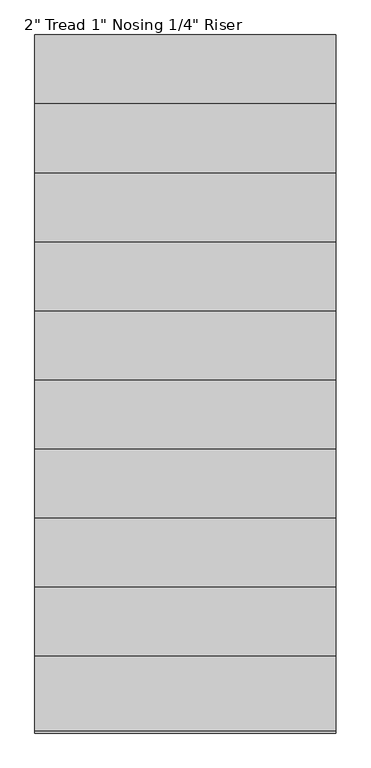
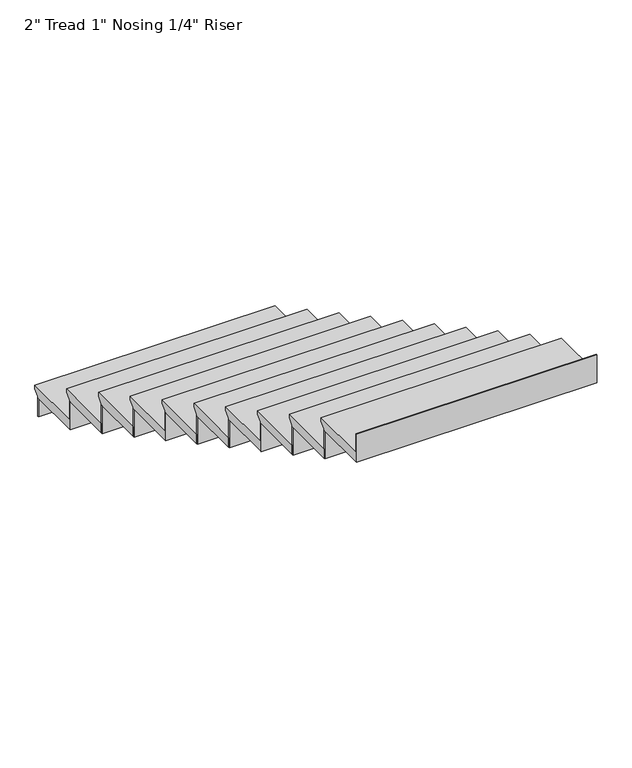
"""IFC4 building model written with IfcOpenShell, lengths in millimetres: stair flight geometry."""

from ifc_helpers import new_model, si_unit, frame, origin, place, context, project, spatial, polyline, outline, extrude, source, transform, mapped, element, save


def stair_flight_d697ccb4(model_context):
    return source(origin(), model_context, "Body", "SweptSolid", [
        extrude(outline(polyline([(11788.0888758, -1500.9090909), (12092.8888758, -1500.9090909), (12092.8888758, -1519.9590909), (12067.4888758, -1545.3590909), (12067.4888758, -1551.7090909), (11788.0888758, -1551.7090909), (11788.0888758, -1500.9090909)])), frame((-1366.3803068, 0.0, 0.0), z_axis=(1.0, 0.0, 0.0), x_axis=(0.0, 1.0, 0.0)), (0.0, 0.0, 1.0), 1219.2),
        extrude(outline(polyline([(-1366.3803068, 12061.1388758), (-1366.3803068, 12067.4888758), (-147.1803068, 12067.4888758), (-147.1803068, 12061.1388758), (-1366.3803068, 12061.1388758)])), frame((0.0, 0.0, -1651.0), z_axis=(0.0, 0.0, 1.0), x_axis=(1.0, 0.0, 0.0)), (0.0, 0.0, 1.0), 99.2909091),
        extrude(outline(polyline([(11508.6888758, -1350.8181818), (11813.4888758, -1350.8181818), (11813.4888758, -1369.8681818), (11788.0888758, -1395.2681818), (11788.0888758, -1401.6181818), (11508.6888758, -1401.6181818), (11508.6888758, -1350.8181818)])), frame((-1366.3803068, 0.0, 0.0), z_axis=(1.0, 0.0, 0.0), x_axis=(0.0, 1.0, 0.0)), (0.0, 0.0, 1.0), 1219.2),
        extrude(outline(polyline([(-1366.3803068, 11781.7388758), (-1366.3803068, 11788.0888758), (-147.1803068, 11788.0888758), (-147.1803068, 11781.7388758), (-1366.3803068, 11781.7388758)])), frame((0.0, 0.0, -1551.7090909), z_axis=(0.0, 0.0, 1.0), x_axis=(1.0, 0.0, 0.0)), (0.0, 0.0, 1.0), 150.0909091),
        extrude(outline(polyline([(11229.2888758, -1200.7272727), (11534.0888758, -1200.7272727), (11534.0888758, -1219.7772727), (11508.6888758, -1245.1772727), (11508.6888758, -1251.5272727), (11229.2888758, -1251.5272727), (11229.2888758, -1200.7272727)])), frame((-1366.3803068, 0.0, 0.0), z_axis=(1.0, 0.0, 0.0), x_axis=(0.0, 1.0, 0.0)), (0.0, 0.0, 1.0), 1219.2),
        extrude(outline(polyline([(-1366.3803068, 11502.3388758), (-1366.3803068, 11508.6888758), (-147.1803068, 11508.6888758), (-147.1803068, 11502.3388758), (-1366.3803068, 11502.3388758)])), frame((0.0, 0.0, -1401.6181818), z_axis=(0.0, 0.0, 1.0), x_axis=(1.0, 0.0, 0.0)), (0.0, 0.0, 1.0), 150.0909091),
        extrude(outline(polyline([(10949.8888758, -1050.6363636), (11254.6888758, -1050.6363636), (11254.6888758, -1069.6863636), (11229.2888758, -1095.0863636), (11229.2888758, -1101.4363636), (10949.8888758, -1101.4363636), (10949.8888758, -1050.6363636)])), frame((-1366.3803068, 0.0, 0.0), z_axis=(1.0, 0.0, 0.0), x_axis=(0.0, 1.0, 0.0)), (0.0, 0.0, 1.0), 1219.2),
        extrude(outline(polyline([(-1366.3803068, 11222.9388758), (-1366.3803068, 11229.2888758), (-147.1803068, 11229.2888758), (-147.1803068, 11222.9388758), (-1366.3803068, 11222.9388758)])), frame((0.0, 0.0, -1251.5272727), z_axis=(0.0, 0.0, 1.0), x_axis=(1.0, 0.0, 0.0)), (0.0, 0.0, 1.0), 150.0909091),
        extrude(outline(polyline([(10670.4888758, -900.5454545), (10975.2888758, -900.5454545), (10975.2888758, -919.5954545), (10949.8888758, -944.9954545), (10949.8888758, -951.3454545), (10670.4888758, -951.3454545), (10670.4888758, -900.5454545)])), frame((-1366.3803068, 0.0, 0.0), z_axis=(1.0, 0.0, 0.0), x_axis=(0.0, 1.0, 0.0)), (0.0, 0.0, 1.0), 1219.2),
        extrude(outline(polyline([(-1366.3803068, 10943.5388758), (-1366.3803068, 10949.8888758), (-147.1803068, 10949.8888758), (-147.1803068, 10943.5388758), (-1366.3803068, 10943.5388758)])), frame((0.0, 0.0, -1101.4363636), z_axis=(0.0, 0.0, 1.0), x_axis=(1.0, 0.0, 0.0)), (0.0, 0.0, 1.0), 150.0909091),
        extrude(outline(polyline([(10391.0888758, -750.4545455), (10695.8888758, -750.4545455), (10695.8888758, -769.5045455), (10670.4888758, -794.9045455), (10670.4888758, -801.2545455), (10391.0888758, -801.2545455), (10391.0888758, -750.4545455)])), frame((-1366.3803068, 0.0, 0.0), z_axis=(1.0, 0.0, 0.0), x_axis=(0.0, 1.0, 0.0)), (0.0, 0.0, 1.0), 1219.2),
        extrude(outline(polyline([(-1366.3803068, 10664.1388758), (-1366.3803068, 10670.4888758), (-147.1803068, 10670.4888758), (-147.1803068, 10664.1388758), (-1366.3803068, 10664.1388758)])), frame((0.0, 0.0, -951.3454545), z_axis=(0.0, 0.0, 1.0), x_axis=(1.0, 0.0, 0.0)), (0.0, 0.0, 1.0), 150.0909091),
        extrude(outline(polyline([(10111.6888758, -600.3636364), (10416.4888758, -600.3636364), (10416.4888758, -619.4136364), (10391.0888758, -644.8136364), (10391.0888758, -651.1636364), (10111.6888758, -651.1636364), (10111.6888758, -600.3636364)])), frame((-1366.3803068, 0.0, 0.0), z_axis=(1.0, 0.0, 0.0), x_axis=(0.0, 1.0, 0.0)), (0.0, 0.0, 1.0), 1219.2),
        extrude(outline(polyline([(-1366.3803068, 10384.7388758), (-1366.3803068, 10391.0888758), (-147.1803068, 10391.0888758), (-147.1803068, 10384.7388758), (-1366.3803068, 10384.7388758)])), frame((0.0, 0.0, -801.2545455), z_axis=(0.0, 0.0, 1.0), x_axis=(1.0, 0.0, 0.0)), (0.0, 0.0, 1.0), 150.0909091),
        extrude(outline(polyline([(9832.2888758, -450.2727273), (10137.0888758, -450.2727273), (10137.0888758, -469.3227273), (10111.6888758, -494.7227273), (10111.6888758, -501.0727273), (9832.2888758, -501.0727273), (9832.2888758, -450.2727273)])), frame((-1366.3803068, 0.0, 0.0), z_axis=(1.0, 0.0, 0.0), x_axis=(0.0, 1.0, 0.0)), (0.0, 0.0, 1.0), 1219.2),
        extrude(outline(polyline([(-1366.3803068, 10105.3388758), (-1366.3803068, 10111.6888758), (-147.1803068, 10111.6888758), (-147.1803068, 10105.3388758), (-1366.3803068, 10105.3388758)])), frame((0.0, 0.0, -651.1636364), z_axis=(0.0, 0.0, 1.0), x_axis=(1.0, 0.0, 0.0)), (0.0, 0.0, 1.0), 150.0909091),
        extrude(outline(polyline([(9552.8888758, -300.1818182), (9857.6888758, -300.1818182), (9857.6888758, -319.2318182), (9832.2888758, -344.6318182), (9832.2888758, -350.9818182), (9552.8888758, -350.9818182), (9552.8888758, -300.1818182)])), frame((-1366.3803068, 0.0, 0.0), z_axis=(1.0, 0.0, 0.0), x_axis=(0.0, 1.0, 0.0)), (0.0, 0.0, 1.0), 1219.2),
        extrude(outline(polyline([(-1366.3803068, 9825.9388758), (-1366.3803068, 9832.2888758), (-147.1803068, 9832.2888758), (-147.1803068, 9825.9388758), (-1366.3803068, 9825.9388758)])), frame((0.0, 0.0, -501.0727273), z_axis=(0.0, 0.0, 1.0), x_axis=(1.0, 0.0, 0.0)), (0.0, 0.0, 1.0), 150.0909091),
        extrude(outline(polyline([(9273.4888758, -150.0909091), (9578.2888758, -150.0909091), (9578.2888758, -169.1409091), (9552.8888758, -194.5409091), (9552.8888758, -200.8909091), (9273.4888758, -200.8909091), (9273.4888758, -150.0909091)])), frame((-1366.3803068, 0.0, 0.0), z_axis=(1.0, 0.0, 0.0), x_axis=(0.0, 1.0, 0.0)), (0.0, 0.0, 1.0), 1219.2),
        extrude(outline(polyline([(-1366.3803068, 9546.5388758), (-1366.3803068, 9552.8888758), (-147.1803068, 9552.8888758), (-147.1803068, 9546.5388758), (-1366.3803068, 9546.5388758)])), frame((0.0, 0.0, -350.9818182), z_axis=(0.0, 0.0, 1.0), x_axis=(1.0, 0.0, 0.0)), (0.0, 0.0, 1.0), 150.0909091),
        extrude(outline(polyline([(-1366.3803068, 9267.1388758), (-1366.3803068, 9273.4888758), (-147.1803068, 9273.4888758), (-147.1803068, 9267.1388758), (-1366.3803068, 9267.1388758)])), frame((0.0, 0.0, -200.8909091), z_axis=(0.0, 0.0, 1.0), x_axis=(1.0, 0.0, 0.0)), (0.0, 0.0, 1.0), 150.0909091),
    ])


if __name__ == "__main__":
    model = new_model("IFC4")
    model_context = context("Model", 3, world=origin())
    ifc_project = project(units=[si_unit("LENGTHUNIT", "METRE", prefix="MILLI")], contexts=[model_context])
    site = spatial("IfcSite", under=ifc_project)
    building = spatial("IfcBuilding", under=site)
    placement = place(None, origin())
    stair_flight_shape = stair_flight_d697ccb4(model_context)
    element("IfcStairFlight", 1, ObjectType="2\" Tread 1\" Nosing 1/4\" Riser", at=placement, inside=building, context=model_context, shape_type="MappedRepresentation", body=[
        mapped(stair_flight_shape, transform((0.0, 0.0, 0.0), x_axis=(1.0, 0.0, 0.0), y_axis=(0.0, 1.0, 0.0), z_axis=(0.0, 0.0, 1.0))),
    ])
    save(model, "model.ifc")

# Revit data of these elements
# Element 1 (IfcStairFlight, "2\" Tread 1\" Nosing 1/4\" Riser")
#   Materials on its faces: "Oak Flooring"
# Materials
#   "Oak Flooring": class "Wood", colour RGB 216 169 114, transparency 0, Description = "Quercus Rubra", Cost = 0
